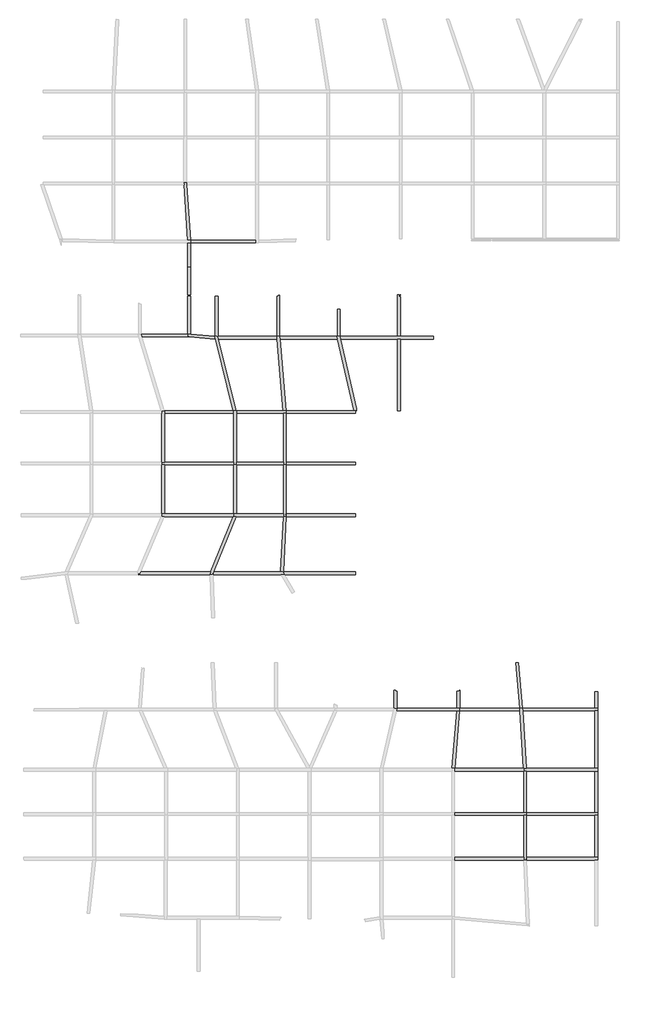
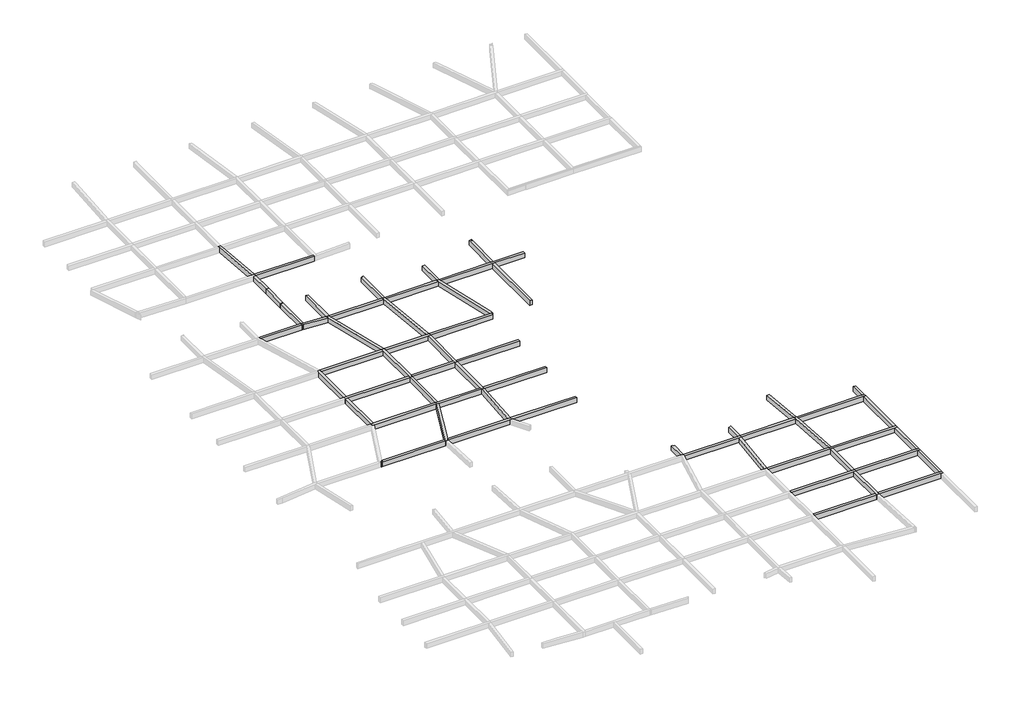
# One storey, part 14 of 15: 57 beams.
"""IFC4 building model written with IfcOpenShell, lengths in millimetres."""

from ifc_helpers import new_model, si_unit, frame, origin, place, context, project, spatial, polyline, outline, extrude, faceted_brep, element, save

model = new_model("IFC4")

# Units and contexts
model_context = context("Model", 3, world=origin())
ifc_project = project(units=[si_unit("LENGTHUNIT", "METRE", prefix="MILLI")], contexts=[model_context])

# Site, building, storey
site = spatial("IfcSite", under=ifc_project)
building = spatial("IfcBuilding", under=site)
storey = spatial("IfcBuildingStorey", under=building, Name="层高", Elevation=3300.0)

# Beams
placement = place(None, origin())
element("IfcBeam", 1, ObjectType="混凝土 - 矩形梁 : KL_beam", at=placement, inside=storey, context=model_context, shape_type="Brep", body=[
    faceted_brep([(295749.8189959, 38242.26105, 3300.0), (295749.8189959, 38542.26105, 3300.0), (295449.8189959, 38542.26105, 3300.0), (287949.8189959, 38542.26105, 3300.0), (287949.8189959, 38242.26105, 3300.0), (295449.8189959, 38242.26105, 3300.0), (295749.8189959, 38242.26105, 2700.0), (287949.8189959, 38242.26105, 2700.0), (295449.8189959, 38242.26105, 2700.0), (295749.8189959, 38542.26105, 2700.0), (287949.8189959, 38542.26105, 2700.0), (295449.8189959, 38542.26105, 2700.0)], [[[0, 1, 2, 3, 4, 5]], [[6, 0, 5, 4, 7, 8]], [[9, 6, 8, 7, 10, 11]], [[1, 9, 11, 10, 3, 2]], [[4, 3, 10, 7]], [[1, 0, 6, 9]]]),
])
element("IfcBeam", 2, ObjectType="混凝土 - 矩形梁 : KL_beam", at=placement, inside=storey, context=model_context, shape_type="Brep", body=[
    faceted_brep([(295449.8189959, 33392.26105, 3300.0), (295456.3366783, 33392.26105, 3300.0), (295749.8189959, 33392.26105, 3300.0), (295749.8189959, 33545.5922638, 3300.0), (295749.8189959, 33692.26105, 3300.0), (295749.8189959, 38242.26105, 3300.0), (295449.8189959, 38242.26105, 3300.0), (295449.8189959, 33692.26105, 3300.0), (295449.8189959, 33392.26105, 2700.0), (295449.8189959, 38242.26105, 2700.0), (295449.8189959, 33692.26105, 2700.0), (295749.8189959, 33392.26105, 2700.0), (295456.3366783, 33392.26105, 2700.0), (295749.8189959, 38242.26105, 2700.0), (295749.8189959, 33692.26105, 2700.0), (295749.8189959, 33545.5922638, 2700.0)], [[[0, 1, 2, 3, 4, 5, 6, 7]], [[8, 0, 7, 6, 9, 10]], [[11, 12, 8, 10, 9, 13, 14, 15]], [[2, 11, 15, 14, 13, 5, 4, 3]], [[6, 5, 13, 9]], [[2, 1, 0, 8, 12, 11]]]),
])
element("IfcBeam", 3, ObjectType="混凝土 - 矩形梁 : KL_beam", at=placement, inside=storey, context=model_context, shape_type="SweptSolid", body=[
    extrude(outline(polyline([(287949.8189959, 33392.26105), (287949.8189959, 33692.26105), (295449.8189959, 33692.26105), (295449.8189959, 33392.26105), (287949.8189959, 33392.26105)])), frame((0.0, 0.0, 2700.0), z_axis=(0.0, 0.0, 1.0), x_axis=(1.0, 0.0, 0.0)), (0.0, 0.0, 1.0), 600.0),
])
element("IfcBeam", 4, ObjectType="混凝土 - 矩形梁 : KL_beam", at=placement, inside=storey, context=model_context, shape_type="Brep", body=[
    faceted_brep([(288493.1023865, 49901.7141002, 3300.0), (288493.1023865, 49901.7141002, 2700.0), (288205.2674175, 49901.7141002, 2700.0), (281663.9582145, 49901.7141002, 2700.0), (281394.6387533, 49901.7141002, 2700.0), (281394.6387533, 49901.7141002, 3300.0), (281663.9582145, 49901.7141002, 3300.0), (288205.2674175, 49901.7141002, 3300.0), (288493.1023865, 49601.7141002, 3300.0), (288192.0287258, 49601.7141002, 3300.0), (281633.2776757, 49601.7141002, 3300.0), (281633.2776757, 49601.7141002, 2700.0), (288192.0287258, 49601.7141002, 2700.0), (288493.1023865, 49601.7141002, 2700.0), (281686.9520176, 49834.2385082, 3300.0), (281686.9520176, 49834.2385082, 2700.0)], [[[0, 1, 2, 3, 4, 5, 6, 7]], [[8, 9, 10, 11, 12, 13]], [[14, 15, 11, 10]], [[15, 14, 5, 4]], [[8, 13, 1, 0]], [[10, 9, 8, 0, 7, 6, 5, 14]], [[13, 12, 11, 15, 4, 3, 2, 1]]]),
])
element("IfcBeam", 5, ObjectType="混凝土 - 矩形梁 : KL_beam", at=placement, inside=storey, context=model_context, shape_type="Brep", body=[
    faceted_brep([(303499.820949, 33392.26105, 3300.0), (303499.820949, 33692.26105, 3300.0), (303199.820949, 33692.26105, 3300.0), (295749.8189959, 33692.26105, 3300.0), (295749.8189959, 33545.5922638, 3300.0), (295756.6327439, 33392.26105, 3300.0), (303199.820949, 33392.26105, 3300.0), (303499.820949, 33392.26105, 2700.0), (295756.6327439, 33392.26105, 2700.0), (303199.820949, 33392.26105, 2700.0), (303499.820949, 33692.26105, 2700.0), (295749.8189959, 33545.5922638, 2700.0), (295749.8189959, 33692.26105, 2700.0), (303199.820949, 33692.26105, 2700.0)], [[[0, 1, 2, 3, 4, 5, 6]], [[7, 0, 6, 5, 8, 9]], [[10, 7, 9, 8, 11, 12, 13]], [[12, 3, 2, 1, 10, 13]], [[3, 12, 11, 4]], [[5, 4, 11, 8]], [[1, 0, 7, 10]]]),
])
element("IfcBeam", 6, ObjectType="混凝土 - 矩形梁 : KL_beam", at=placement, inside=storey, context=model_context, shape_type="Brep", body=[
    faceted_brep([(303499.820949, 38242.26105, 3300.0), (303499.820949, 38542.26105, 3300.0), (303199.820949, 38542.26105, 3300.0), (295749.8189959, 38542.26105, 3300.0), (295749.8189959, 38242.26105, 3300.0), (303199.820949, 38242.26105, 3300.0), (303499.820949, 38242.26105, 2700.0), (295749.8189959, 38242.26105, 2700.0), (303199.820949, 38242.26105, 2700.0), (303499.820949, 38542.26105, 2700.0), (295749.8189959, 38542.26105, 2700.0), (303199.820949, 38542.26105, 2700.0)], [[[0, 1, 2, 3, 4, 5]], [[6, 0, 5, 4, 7, 8]], [[9, 6, 8, 7, 10, 11]], [[1, 9, 11, 10, 3, 2]], [[4, 3, 10, 7]], [[1, 0, 6, 9]]]),
])
element("IfcBeam", 7, ObjectType="混凝土 - 矩形梁 : KL_beam", at=placement, inside=storey, context=model_context, shape_type="Brep", body=[
    faceted_brep([(303499.820949, 43042.26105, 3300.0), (303499.820949, 43342.26105, 3300.0), (303199.820949, 43342.26105, 3300.0), (295740.5303996, 43342.26105, 3300.0), (295449.8189959, 43342.26105, 3300.0), (295449.8189959, 43042.26105, 3300.0), (295749.8189959, 43042.26105, 3300.0), (303199.820949, 43042.26105, 3300.0), (303499.820949, 43042.26105, 2700.0), (295449.8189959, 43042.26105, 2700.0), (295749.8189959, 43042.26105, 2700.0), (303199.820949, 43042.26105, 2700.0), (303499.820949, 43342.26105, 2700.0), (295449.8189959, 43342.26105, 2700.0), (295740.5303996, 43342.26105, 2700.0), (303199.820949, 43342.26105, 2700.0)], [[[0, 1, 2, 3, 4, 5, 6, 7]], [[8, 0, 7, 6, 5, 9, 10, 11]], [[12, 8, 11, 10, 9, 13, 14, 15]], [[1, 12, 15, 14, 13, 4, 3, 2]], [[1, 0, 8, 12]], [[5, 4, 13, 9]]]),
])
element("IfcBeam", 8, ObjectType="混凝土 - 矩形梁 : KL_beam", at=placement, inside=storey, context=model_context, shape_type="SweptSolid", body=[
    extrude(outline(polyline([(303499.820949, 38542.26105), (303199.820949, 38542.26105), (303199.820949, 43042.26105), (303499.820949, 43042.26105), (303499.820949, 38542.26105)])), frame((0.0, 0.0, 2700.0), z_axis=(0.0, 0.0, 1.0), x_axis=(1.0, 0.0, 0.0)), (0.0, 0.0, 1.0), 600.0),
])
element("IfcBeam", 9, ObjectType="混凝土 - 矩形梁 : KL_beam", at=placement, inside=storey, context=model_context, shape_type="SweptSolid", body=[
    extrude(outline(polyline([(295749.8189959, 38542.26105), (295449.8189959, 38542.26105), (295449.8189959, 43042.26105), (295749.8189959, 43042.26105), (295749.8189959, 38542.26105)])), frame((0.0, 0.0, 2700.0), z_axis=(0.0, 0.0, 1.0), x_axis=(1.0, 0.0, 0.0)), (0.0, 0.0, 1.0), 600.0),
])
element("IfcBeam", 10, ObjectType="混凝土 - 矩形梁 : KL_beam", at=placement, inside=storey, context=model_context, shape_type="Brep", body=[
    faceted_brep([(295449.8189959, 43042.26105, 3300.0), (295449.8189959, 43342.26105, 3300.0), (295439.9172438, 43342.26105, 3300.0), (287963.0576876, 43342.26105, 3300.0), (287949.8189959, 43342.26105, 3300.0), (287949.8189959, 43042.26105, 3300.0), (295449.8189959, 43042.26105, 2700.0), (287949.8189959, 43042.26105, 2700.0), (295449.8189959, 43342.26105, 2700.0), (287949.8189959, 43342.26105, 2700.0), (287963.0576876, 43342.26105, 2700.0), (295439.9172438, 43342.26105, 2700.0)], [[[0, 1, 2, 3, 4, 5]], [[6, 0, 5, 7]], [[8, 6, 7, 9, 10, 11]], [[1, 8, 11, 10, 9, 4, 3, 2]], [[1, 0, 6, 8]], [[5, 4, 9, 7]]]),
])
element("IfcBeam", 11, ObjectType="混凝土 - 矩形梁 : KL_beam", at=placement, inside=storey, context=model_context, shape_type="Brep", body=[
    faceted_brep([(288493.1023865, 49601.7141002, 2700.0), (288493.1023865, 49601.7141002, 3300.0), (287963.0576876, 43342.26105, 3300.0), (287963.0576876, 43342.26105, 2700.0), (288192.0287258, 49601.7141002, 3300.0), (288192.0287258, 49601.7141002, 2700.0), (287661.984027, 43342.26105, 3300.0), (287661.984027, 43342.26105, 2700.0), (287949.8189959, 43342.26105, 2700.0), (287949.8189959, 43342.26105, 3300.0)], [[[0, 1, 2, 3]], [[4, 1, 0, 5]], [[6, 7, 8, 3, 2, 9]], [[1, 4, 6, 9, 2]], [[4, 5, 7, 6]], [[5, 0, 3, 8, 7]]]),
])
element("IfcBeam", 12, ObjectType="混凝土 - 矩形梁 : KL_beam", at=placement, inside=storey, context=model_context, shape_type="Brep", body=[
    faceted_brep([(295439.9172438, 43342.26105, 3300.0), (295449.8189959, 43342.26105, 3300.0), (295740.5303996, 43342.26105, 3300.0), (295340.1267819, 49601.7141002, 3300.0), (295320.9364335, 49901.7141002, 3300.0), (295317.6747059, 49901.7141002, 3300.0), (295020.3232776, 49901.7141002, 3300.0), (295039.5136261, 49601.7141002, 3300.0), (295020.3232776, 49901.7141002, 2700.0), (295039.5136261, 49601.7141002, 2700.0), (295439.9172438, 43342.26105, 2700.0), (295740.5303996, 43342.26105, 2700.0), (295449.8189959, 43342.26105, 2700.0), (295317.6747059, 49901.7141002, 2700.0), (295320.9364335, 49901.7141002, 2700.0), (295340.1267819, 49601.7141002, 2700.0)], [[[0, 1, 2, 3, 4, 5, 6, 7]], [[6, 8, 9, 10, 0, 7]], [[11, 12, 10, 9, 8, 13, 14, 15]], [[2, 11, 15, 14, 4, 3]], [[0, 10, 12, 11, 2, 1]], [[6, 5, 4, 14, 13, 8]]]),
])
element("IfcBeam", 13, ObjectType="混凝土 - 矩形梁 : KL_beam", at=placement, inside=storey, context=model_context, shape_type="Brep", body=[
    faceted_brep([(288493.1023865, 49901.7141002, 3300.0), (288493.1023865, 49601.7141002, 3300.0), (295039.5136261, 49601.7141002, 3300.0), (295020.3232776, 49901.7141002, 3300.0), (295016.5287546, 49901.7141002, 3300.0), (288505.2674175, 49901.7141002, 3300.0), (288493.1023865, 49601.7141002, 2700.0), (295039.5136261, 49601.7141002, 2700.0), (288493.1023865, 49901.7141002, 2700.0), (288505.2674175, 49901.7141002, 2700.0), (295016.5287546, 49901.7141002, 2700.0), (295020.3232776, 49901.7141002, 2700.0)], [[[0, 1, 2, 3, 4, 5]], [[1, 6, 7, 2]], [[6, 8, 9, 10, 11, 7]], [[8, 0, 5, 4, 3, 11, 10, 9]], [[1, 0, 8, 6]], [[3, 2, 7, 11]]]),
])
element("IfcBeam", 14, ObjectType="混凝土 - 矩形梁 : KL_beam", at=placement, inside=storey, context=model_context, shape_type="Brep", body=[
    faceted_brep([(295320.9364335, 49901.7141002, 3300.0), (295340.1267819, 49601.7141002, 3300.0), (303199.820949, 49601.7141002, 3300.0), (303499.820949, 49601.7141002, 3300.0), (303499.820949, 49901.7141002, 3300.0), (303199.820949, 49901.7141002, 3300.0), (295340.1267819, 49601.7141002, 2700.0), (303199.820949, 49601.7141002, 2700.0), (303499.820949, 49601.7141002, 2700.0), (295320.9364335, 49901.7141002, 2700.0), (303199.820949, 49901.7141002, 2700.0), (303499.820949, 49901.7141002, 2700.0)], [[[0, 1, 2, 3, 4, 5]], [[1, 6, 7, 8, 3, 2]], [[6, 9, 10, 11, 8, 7]], [[9, 0, 5, 4, 11, 10]], [[1, 0, 9, 6]], [[4, 3, 8, 11]]]),
])
element("IfcBeam", 15, ObjectType="混凝土 - 矩形梁 : KL_beam", at=placement, inside=storey, context=model_context, shape_type="SweptSolid", body=[
    extrude(outline(polyline([(303499.820949, 43342.26105), (303199.820949, 43342.26105), (303199.820949, 49601.7141002), (303499.820949, 49601.7141002), (303499.820949, 43342.26105)])), frame((0.0, 0.0, 2700.0), z_axis=(0.0, 0.0, 1.0), x_axis=(1.0, 0.0, 0.0)), (0.0, 0.0, 1.0), 600.0),
])
element("IfcBeam", 16, ObjectType="混凝土 - 矩形梁 : KL_beam", at=placement, inside=storey, context=model_context, shape_type="SweptSolid", body=[
    extrude(outline(polyline([(303499.820949, 49901.7141002), (303199.820949, 49901.7141002), (303199.820949, 51682.3314613), (303499.820949, 51682.3314613), (303499.820949, 49901.7141002)])), frame((0.0, 0.0, 2700.0), z_axis=(0.0, 0.0, 1.0), x_axis=(1.0, 0.0, 0.0)), (0.0, 0.0, 1.0), 600.0),
])
element("IfcBeam", 17, ObjectType="混凝土 - 矩形梁 : KL_beam", at=placement, inside=storey, context=model_context, shape_type="Brep", body=[
    faceted_brep([(281363.9582145, 51842.0227808, 2700.0), (281363.9582145, 51842.0227808, 3300.0), (281540.2344711, 51842.0227808, 3300.0), (281540.2344711, 51842.0227808, 2700.0), (281363.9582145, 49901.7141002, 3300.0), (281394.6387533, 49901.7141002, 3300.0), (281663.9582145, 49901.7141002, 3300.0), (281663.9582145, 51732.3246977, 3300.0), (281540.2344711, 51732.3246977, 3300.0), (281663.9582145, 49901.7141002, 2700.0), (281663.9582145, 51732.3246977, 2700.0), (281363.9582145, 49901.7141002, 2700.0), (281540.2344711, 51732.3246977, 2700.0), (281394.6387533, 49901.7141002, 2700.0)], [[[0, 1, 2, 3]], [[1, 4, 5, 6, 7, 8, 2]], [[6, 9, 10, 7]], [[11, 0, 3, 12, 10, 9, 13]], [[1, 0, 11, 4]], [[4, 11, 13, 9, 6, 5]], [[12, 8, 7, 10]], [[8, 12, 3, 2]]]),
])
element("IfcBeam", 18, ObjectType="混凝土 - 矩形梁 : KL_beam", at=placement, inside=storey, context=model_context, shape_type="Brep", body=[
    faceted_brep([(288205.2674175, 49901.7141002, 3300.0), (288493.1023865, 49901.7141002, 3300.0), (288505.2674175, 49901.7141002, 3300.0), (288505.2674175, 51852.3246977, 3300.0), (288460.2344711, 51852.3246977, 3300.0), (288460.2344711, 51732.3246977, 3300.0), (288340.2344711, 51732.3246977, 3300.0), (288205.2674175, 51732.3246977, 3300.0), (288505.2674175, 49901.7141002, 2700.0), (288505.2674175, 51852.3246977, 2700.0), (288493.1023865, 49901.7141002, 2700.0), (288205.2674175, 49901.7141002, 2700.0), (288205.2674175, 51732.3246977, 2700.0), (288460.2344711, 51732.3246977, 2700.0), (288460.2344711, 51852.3246977, 2700.0)], [[[0, 1, 2, 3, 4, 5, 6, 7]], [[2, 8, 9, 3]], [[8, 10, 11, 12, 13, 14, 9]], [[11, 0, 7, 12]], [[0, 11, 10, 8, 2, 1]], [[3, 9, 14, 4]], [[5, 13, 12, 7, 6]], [[13, 5, 4, 14]]]),
])
element("IfcBeam", 19, ObjectType="混凝土 - 矩形梁 : KL_beam", at=placement, inside=storey, context=model_context, shape_type="Brep", body=[
    faceted_brep([(295016.5287546, 49901.7141002, 3300.0), (295020.3232776, 49901.7141002, 3300.0), (295317.6747059, 49901.7141002, 3300.0), (294886.3021743, 54832.3246977, 3300.0), (294585.1562231, 54832.3246977, 3300.0), (295317.6747059, 49901.7141002, 2700.0), (294886.3021743, 54832.3246977, 2700.0), (295020.3232776, 49901.7141002, 2700.0), (295016.5287546, 49901.7141002, 2700.0), (294585.1562231, 54832.3246977, 2700.0)], [[[0, 1, 2, 3, 4]], [[2, 5, 6, 3]], [[5, 7, 8, 9, 6]], [[8, 0, 4, 9]], [[5, 2, 1, 0, 8, 7]], [[4, 3, 6, 9]]]),
])
element("IfcBeam", 20, ObjectType="混凝土 - 矩形梁 : KL_beam", at=placement, inside=storey, context=model_context, shape_type="SweptSolid", body=[
    extrude(outline(polyline([(303499.820949, 33692.26105), (303199.820949, 33692.26105), (303199.820949, 38242.26105), (303499.820949, 38242.26105), (303499.820949, 33692.26105)])), frame((0.0, 0.0, 2700.0), z_axis=(0.0, 0.0, 1.0), x_axis=(1.0, 0.0, 0.0)), (0.0, 0.0, 1.0), 600.0),
])
element("IfcBeam", 21, ObjectType="混凝土 - 矩形梁 : KL_beam", at=placement, inside=storey, context=model_context, shape_type="SweptSolid", body=[
    extrude(outline(polyline([(259271.6890495, 97741.6486698), (258971.6890495, 97741.6486698), (258971.6890495, 100391.6486698), (259271.6890495, 100391.6486698), (259271.6890495, 97741.6486698)])), frame((0.0, 0.0, 2700.0), z_axis=(0.0, 0.0, 1.0), x_axis=(1.0, 0.0, 0.0)), (0.0, 0.0, 1.0), 600.0),
])
element("IfcBeam", 22, ObjectType="混凝土 - 矩形梁 : KL_beam", at=placement, inside=storey, context=model_context, shape_type="Brep", body=[
    faceted_brep([(263949.8021775, 76292.0126466, 3300.0), (264249.8021775, 76292.0126466, 3300.0), (264249.8021775, 76592.0126466, 3300.0), (264249.8021775, 81892.0126467, 3300.0), (264249.8021775, 82192.0126467, 3300.0), (264216.9950214, 82192.0126467, 3300.0), (263949.8021775, 82192.0126467, 3300.0), (263949.8021775, 81892.0126467, 3300.0), (263949.8021775, 76592.0126466, 3300.0), (263949.8021775, 76292.0126466, 2700.0), (263949.8021775, 82192.0126467, 2700.0), (263949.8021775, 81892.0126467, 2700.0), (263949.8021775, 76592.0126466, 2700.0), (264249.8021775, 76292.0126466, 2700.0), (264216.9950214, 82192.0126467, 2700.0), (264249.8021775, 82192.0126467, 2700.0), (264249.8021775, 81892.0126467, 2700.0), (264249.8021775, 76592.0126466, 2700.0)], [[[0, 1, 2, 3, 4, 5, 6, 7, 8]], [[9, 0, 8, 7, 6, 10, 11, 12]], [[13, 9, 12, 11, 10, 14, 15, 16, 17]], [[1, 13, 17, 16, 15, 4, 3, 2]], [[1, 0, 9, 13]], [[6, 5, 4, 15, 14, 10]]]),
])
element("IfcBeam", 23, ObjectType="混凝土 - 矩形梁 : KL_beam", at=placement, inside=storey, context=model_context, shape_type="Brep", body=[
    faceted_brep([(256149.8021771, 76592.0126466, 3300.0), (256149.8021771, 76302.5702379, 3300.0), (256149.8021771, 76292.0126466, 3300.0), (256449.8021771, 76292.0126466, 3300.0), (263949.8021775, 76292.0126466, 3300.0), (263949.8021775, 76592.0126466, 3300.0), (256449.8021771, 76592.0126466, 3300.0), (256149.8021771, 76592.0126466, 2700.0), (263949.8021775, 76592.0126466, 2700.0), (256449.8021771, 76592.0126466, 2700.0), (256149.8021771, 76292.0126466, 2700.0), (256149.8021771, 76302.5702379, 2700.0), (263949.8021775, 76292.0126466, 2700.0), (256449.8021771, 76292.0126466, 2700.0)], [[[0, 1, 2, 3, 4, 5, 6]], [[7, 0, 6, 5, 8, 9]], [[10, 11, 7, 9, 8, 12, 13]], [[2, 10, 13, 12, 4, 3]], [[5, 4, 12, 8]], [[2, 1, 0, 7, 11, 10]]]),
])
element("IfcBeam", 24, ObjectType="混凝土 - 矩形梁 : KL_beam", at=placement, inside=storey, context=model_context, shape_type="Brep", body=[
    faceted_brep([(256449.8021771, 82192.0126467, 3300.0), (256410.7963384, 82192.0126467, 3300.0), (256149.8021771, 82192.0126467, 3300.0), (256149.8021771, 82019.5949965, 3300.0), (256149.8021771, 81897.4603606, 3300.0), (256149.8021771, 76602.5702379, 3300.0), (256149.8021771, 76592.0126466, 3300.0), (256449.8021771, 76592.0126466, 3300.0), (256449.8021771, 81892.0126467, 3300.0), (256149.8021771, 82192.0126467, 2700.0), (256149.8021771, 82019.5949965, 2700.0), (256149.8021771, 81897.4603606, 2700.0), (256149.8021771, 76602.5702379, 2700.0), (256149.8021771, 76592.0126466, 2700.0), (256410.7963384, 82192.0126467, 2700.0), (256449.8021771, 82192.0126467, 2700.0), (256449.8021771, 81892.0126467, 2700.0), (256449.8021771, 76592.0126466, 2700.0)], [[[0, 1, 2, 3, 4, 5, 6, 7, 8]], [[2, 9, 10, 11, 12, 13, 6, 5, 4, 3]], [[9, 14, 15, 16, 17, 13, 12, 11, 10]], [[15, 0, 8, 7, 17, 16]], [[7, 6, 13, 17]], [[2, 1, 0, 15, 14, 9]]]),
])
element("IfcBeam", 25, ObjectType="混凝土 - 矩形梁 : KL_beam", at=placement, inside=storey, context=model_context, shape_type="Brep", body=[
    faceted_brep([(263949.8021775, 81892.0126467, 3300.0), (263949.8021775, 82192.0126467, 3300.0), (263907.8109326, 82192.0126467, 3300.0), (256449.8021771, 82192.0126467, 3300.0), (256449.8021771, 81892.0126467, 3300.0), (263949.8021775, 81892.0126467, 2700.0), (256449.8021771, 81892.0126467, 2700.0), (263949.8021775, 82192.0126467, 2700.0), (256449.8021771, 82192.0126467, 2700.0), (263907.8109326, 82192.0126467, 2700.0)], [[[0, 1, 2, 3, 4]], [[5, 0, 4, 6]], [[7, 5, 6, 8, 9]], [[1, 7, 9, 8, 3, 2]], [[1, 0, 5, 7]], [[4, 3, 8, 6]]]),
])
element("IfcBeam", 26, ObjectType="混凝土 - 矩形梁 : KL_beam", at=placement, inside=storey, context=model_context, shape_type="Brep", body=[
    faceted_brep([(264249.8021775, 82192.0126467, 3300.0), (264249.8021775, 81892.0126467, 3300.0), (269354.7419848, 81892.0126467, 3300.0), (269654.7419848, 81892.0126467, 3300.0), (269654.7419848, 82192.0126467, 3300.0), (269642.1916609, 82192.0126467, 3300.0), (269341.0457096, 82192.0126467, 3300.0), (264249.8021775, 81892.0126467, 2700.0), (269354.7419848, 81892.0126467, 2700.0), (269654.7419848, 81892.0126467, 2700.0), (264249.8021775, 82192.0126467, 2700.0), (269341.0457096, 82192.0126467, 2700.0), (269642.1916609, 82192.0126467, 2700.0), (269654.7419848, 82192.0126467, 2700.0)], [[[0, 1, 2, 3, 4, 5, 6]], [[1, 7, 8, 9, 3, 2]], [[7, 10, 11, 12, 13, 9, 8]], [[10, 0, 6, 5, 4, 13, 12, 11]], [[1, 0, 10, 7]], [[4, 3, 9, 13]]]),
])
element("IfcBeam", 27, ObjectType="混凝土 - 矩形梁 : KL_beam", at=placement, inside=storey, context=model_context, shape_type="Brep", body=[
    faceted_brep([(269354.7419848, 76292.0126466, 3300.0), (269654.7419848, 76292.0126466, 3300.0), (269654.7419848, 76592.0126466, 3300.0), (269654.7419848, 81892.0126467, 3300.0), (269354.7419848, 81892.0126467, 3300.0), (269354.7419848, 76592.0126466, 3300.0), (269354.7419848, 76292.0126466, 2700.0), (269354.7419848, 81892.0126467, 2700.0), (269354.7419848, 76592.0126466, 2700.0), (269654.7419848, 76292.0126466, 2700.0), (269654.7419848, 81892.0126467, 2700.0), (269654.7419848, 76592.0126466, 2700.0)], [[[0, 1, 2, 3, 4, 5]], [[6, 0, 5, 4, 7, 8]], [[9, 6, 8, 7, 10, 11]], [[1, 9, 11, 10, 3, 2]], [[4, 3, 10, 7]], [[1, 0, 6, 9]]]),
])
element("IfcBeam", 28, ObjectType="混凝土 - 矩形梁 : KL_beam", at=placement, inside=storey, context=model_context, shape_type="SweptSolid", body=[
    extrude(outline(polyline([(264249.8021775, 76292.0126466), (264249.8021775, 76592.0126466), (269354.7419848, 76592.0126466), (269354.7419848, 76292.0126466), (264249.8021775, 76292.0126466)])), frame((0.0, 0.0, 2700.0), z_axis=(0.0, 0.0, 1.0), x_axis=(1.0, 0.0, 0.0)), (0.0, 0.0, 1.0), 600.0),
])
element("IfcBeam", 29, ObjectType="混凝土 - 矩形梁 : KL_beam", at=placement, inside=storey, context=model_context, shape_type="Brep", body=[
    faceted_brep([(269354.7419848, 70692.0126466, 3300.0), (269647.6593001, 70692.0126466, 3300.0), (269654.7419848, 70692.0126466, 3300.0), (269654.7419848, 70838.3856753, 3300.0), (269654.7419848, 70992.0126466, 3300.0), (269654.7419848, 76292.0126466, 3300.0), (269354.7419848, 76292.0126466, 3300.0), (269354.7419848, 70992.0126466, 3300.0), (269354.7419848, 70692.0126466, 2700.0), (269354.7419848, 76292.0126466, 2700.0), (269354.7419848, 70992.0126466, 2700.0), (269654.7419848, 70692.0126466, 2700.0), (269647.6593001, 70692.0126466, 2700.0), (269654.7419848, 76292.0126466, 2700.0), (269654.7419848, 70992.0126466, 2700.0), (269654.7419848, 70838.3856753, 2700.0)], [[[0, 1, 2, 3, 4, 5, 6, 7]], [[8, 0, 7, 6, 9, 10]], [[11, 12, 8, 10, 9, 13, 14, 15]], [[2, 11, 15, 14, 13, 5, 4, 3]], [[6, 5, 13, 9]], [[2, 1, 0, 8, 12, 11]]]),
])
element("IfcBeam", 30, ObjectType="混凝土 - 矩形梁 : KL_beam", at=placement, inside=storey, context=model_context, shape_type="Brep", body=[
    faceted_brep([(263949.8021775, 70992.0126466, 3300.0), (263949.8021775, 70692.0126466, 3300.0), (264200.978455, 70692.0126466, 3300.0), (269347.308297, 70692.0126466, 3300.0), (269354.7419848, 70692.0126466, 3300.0), (269354.7419848, 70992.0126466, 3300.0), (264249.8021775, 70992.0126466, 3300.0), (263949.8021775, 70992.0126466, 2700.0), (269354.7419848, 70992.0126466, 2700.0), (264249.8021775, 70992.0126466, 2700.0), (263949.8021775, 70692.0126466, 2700.0), (269354.7419848, 70692.0126466, 2700.0), (269347.308297, 70692.0126466, 2700.0), (264200.978455, 70692.0126466, 2700.0)], [[[0, 1, 2, 3, 4, 5, 6]], [[7, 0, 6, 5, 8, 9]], [[10, 7, 9, 8, 11, 12, 13]], [[1, 10, 13, 12, 11, 4, 3, 2]], [[5, 4, 11, 8]], [[1, 0, 7, 10]]]),
])
element("IfcBeam", 31, ObjectType="混凝土 - 矩形梁 : KL_beam", at=placement, inside=storey, context=model_context, shape_type="SweptSolid", body=[
    extrude(outline(polyline([(263949.8021775, 76292.0126466), (264249.8021775, 76292.0126466), (264249.8021775, 70992.0126466), (263949.8021775, 70992.0126466), (263949.8021775, 76292.0126466)])), frame((0.0, 0.0, 2700.0), z_axis=(0.0, 0.0, 1.0), x_axis=(1.0, 0.0, 0.0)), (0.0, 0.0, 1.0), 600.0),
])
element("IfcBeam", 32, ObjectType="混凝土 - 矩形梁 : KL_beam", at=placement, inside=storey, context=model_context, shape_type="Brep", body=[
    faceted_brep([(256149.8021771, 70992.0126466, 3300.0), (256149.8021771, 70872.8035797, 3300.0), (256149.8021771, 70692.0126466, 3300.0), (256398.7084648, 70692.0126466, 3300.0), (263877.4180322, 70692.0126466, 3300.0), (263949.8021775, 70692.0126466, 3300.0), (263949.8021775, 70992.0126466, 3300.0), (256449.8021771, 70992.0126466, 3300.0), (256149.8021771, 70692.0126466, 2700.0), (256398.7084648, 70692.0126466, 2700.0), (263877.4180322, 70692.0126466, 2700.0), (263949.8021775, 70692.0126466, 2700.0), (256149.8021771, 70872.8035797, 2700.0), (256149.8021771, 70992.0126466, 2700.0), (256449.8021771, 70992.0126466, 2700.0), (263949.8021775, 70992.0126466, 2700.0)], [[[0, 1, 2, 3, 4, 5, 6, 7]], [[2, 8, 9, 10, 11, 5, 4, 3]], [[8, 12, 13, 14, 15, 11, 10, 9]], [[13, 0, 7, 6, 15, 14]], [[6, 5, 11, 15]], [[2, 1, 0, 13, 12, 8]]]),
])
element("IfcBeam", 33, ObjectType="混凝土 - 矩形梁 : KL_beam", at=placement, inside=storey, context=model_context, shape_type="SweptSolid", body=[
    extrude(outline(polyline([(256149.8021771, 76292.0126466), (256449.8021771, 76292.0126466), (256449.8021771, 70992.0126466), (256149.8021771, 70992.0126466), (256149.8021771, 76292.0126466)])), frame((0.0, 0.0, 2700.0), z_axis=(0.0, 0.0, 1.0), x_axis=(1.0, 0.0, 0.0)), (0.0, 0.0, 1.0), 600.0),
])
element("IfcBeam", 34, ObjectType="混凝土 - 矩形梁 : KL_beam", at=placement, inside=storey, context=model_context, shape_type="Brep", body=[
    faceted_brep([(264200.978455, 70692.0126466, 3300.0), (263949.8021775, 70692.0126466, 3300.0), (263877.4180322, 70692.0126466, 3300.0), (261453.2606772, 64692.0126466, 3300.0), (261332.0528094, 64392.0126466, 3300.0), (261409.5836385, 64392.0126466, 3300.0), (261655.6132322, 64392.0126466, 3300.0), (261705.4582963, 64515.3835094, 3300.0), (261776.8211, 64692.0126466, 3300.0), (261332.0528094, 64392.0126466, 2700.0), (263877.4180322, 70692.0126466, 2700.0), (261453.2606772, 64692.0126466, 2700.0), (263949.8021775, 70692.0126466, 2700.0), (264200.978455, 70692.0126466, 2700.0), (261776.8211, 64692.0126466, 2700.0), (261705.4582963, 64515.3835094, 2700.0), (261655.6132322, 64392.0126466, 2700.0), (261409.5836385, 64392.0126466, 2700.0)], [[[0, 1, 2, 3, 4, 5, 6, 7, 8]], [[9, 4, 3, 2, 10, 11]], [[10, 12, 13, 14, 15, 16, 17, 9, 11]], [[13, 0, 8, 7, 6, 16, 15, 14]], [[0, 13, 12, 10, 2, 1]], [[6, 5, 4, 9, 17, 16]]]),
])
element("IfcBeam", 35, ObjectType="混凝土 - 矩形梁 : KL_beam", at=placement, inside=storey, context=model_context, shape_type="SweptSolid", body=[
    extrude(outline(polyline([(261453.2606772, 64692.0126466), (261332.0528094, 64392.0126466), (253809.5875713, 64392.0126466), (253809.5875713, 64542.2610502), (253762.8884968, 64542.2610502), (253827.0729182, 64692.0126466), (261453.2606772, 64692.0126466)])), frame((0.0, 0.0, 2700.0), z_axis=(0.0, 0.0, 1.0), x_axis=(1.0, 0.0, 0.0)), (0.0, 0.0, 1.0), 600.0),
    extrude(outline(polyline([(253599.5848532, 64392.0126466), (253599.5848532, 64542.165729), (253689.5875713, 64503.5900308), (253689.5875713, 64392.0126466), (253599.5848532, 64392.0126466)])), frame((0.0, 0.0, 2700.0), z_axis=(0.0, 0.0, 1.0), x_axis=(1.0, 0.0, 0.0)), (0.0, 0.0, 1.0), 600.0),
])
element("IfcBeam", 36, ObjectType="混凝土 - 矩形梁 : KL_beam", at=placement, inside=storey, context=model_context, shape_type="Brep", body=[
    faceted_brep([(269459.7057839, 64392.0126466, 3300.0), (269351.8545261, 64578.8165049, 3300.0), (269286.5007032, 64692.0126466, 3300.0), (269056.9808475, 64692.0126466, 3300.0), (261776.8211, 64692.0126466, 3300.0), (261705.4582963, 64515.3835094, 3300.0), (261709.7665018, 64392.0126466, 3300.0), (269113.2956224, 64392.0126466, 3300.0), (269459.7057839, 64392.0126466, 2700.0), (261709.7665018, 64392.0126466, 2700.0), (269113.2956224, 64392.0126466, 2700.0), (269286.5007032, 64692.0126466, 2700.0), (269351.8545261, 64578.8165049, 2700.0), (261705.4582963, 64515.3835094, 2700.0), (261776.8211, 64692.0126466, 2700.0), (269056.9808475, 64692.0126466, 2700.0)], [[[0, 1, 2, 3, 4, 5, 6, 7]], [[8, 0, 7, 6, 9, 10]], [[11, 12, 8, 10, 9, 13, 14, 15]], [[14, 4, 3, 2, 11, 15]], [[4, 14, 13, 5]], [[6, 5, 13, 9]], [[2, 1, 0, 8, 12, 11]]]),
])
element("IfcBeam", 37, ObjectType="混凝土 - 矩形梁 : KL_beam", at=placement, inside=storey, context=model_context, shape_type="Brep", body=[
    faceted_brep([(269647.6593001, 70692.0126466, 3300.0), (269354.7419848, 70692.0126466, 3300.0), (269347.308297, 70692.0126466, 3300.0), (269056.9808475, 64692.0126466, 3300.0), (269286.5007032, 64692.0126466, 3300.0), (269351.8545261, 64578.8165049, 3300.0), (269357.3318506, 64692.0126466, 3300.0), (269347.308297, 70692.0126466, 2700.0), (269056.9808475, 64692.0126466, 2700.0), (269354.7419848, 70692.0126466, 2700.0), (269647.6593001, 70692.0126466, 2700.0), (269357.3318506, 64692.0126466, 2700.0), (269351.8545261, 64578.8165049, 2700.0), (269286.5007032, 64692.0126466, 2700.0)], [[[0, 1, 2, 3, 4, 5, 6]], [[2, 7, 8, 3]], [[7, 9, 10, 11, 12, 13, 8]], [[10, 0, 6, 5, 12, 11]], [[0, 10, 9, 7, 2, 1]], [[13, 4, 3, 8]], [[4, 13, 12, 5]]]),
    faceted_brep([(269654.7419848, 70992.0126466, 2700.0), (269654.7419848, 70992.0126466, 3300.0), (269662.1756726, 70992.0126466, 3300.0), (269662.1756726, 70992.0126466, 2700.0), (269654.7419848, 70838.3856753, 3300.0), (269654.7419848, 70838.3856753, 2700.0)], [[[0, 1, 2, 3]], [[4, 1, 0, 5]], [[4, 2, 1]], [[3, 5, 0]], [[2, 4, 5, 3]]]),
])
element("IfcBeam", 38, ObjectType="混凝土 - 矩形梁 : KL_beam", at=placement, inside=storey, context=model_context, shape_type="SweptSolid", body=[
    extrude(outline(polyline([(269654.7419848, 70692.0126466), (269654.7419848, 70838.3856753), (269662.1756726, 70992.0126466), (277178.9838503, 70992.0126466), (277178.9838503, 70692.0126466), (269654.7419848, 70692.0126466)])), frame((0.0, 0.0, 2700.0), z_axis=(0.0, 0.0, 1.0), x_axis=(1.0, 0.0, 0.0)), (0.0, 0.0, 1.0), 600.0),
])
element("IfcBeam", 39, ObjectType="混凝土 - 矩形梁 : KL_beam", at=placement, inside=storey, context=model_context, shape_type="SweptSolid", body=[
    extrude(outline(polyline([(269459.7057839, 64392.0126466), (269351.8545261, 64578.8165049), (269357.3318506, 64692.0126466), (277178.9838503, 64692.0126466), (277178.9838503, 64392.0126466), (269459.7057839, 64392.0126466)])), frame((0.0, 0.0, 2700.0), z_axis=(0.0, 0.0, 1.0), x_axis=(1.0, 0.0, 0.0)), (0.0, 0.0, 1.0), 600.0),
])
element("IfcBeam", 40, ObjectType="混凝土 - 矩形梁 : KL_beam", at=placement, inside=storey, context=model_context, shape_type="SweptSolid", body=[
    extrude(outline(polyline([(269654.7419848, 76292.0126466), (269654.7419848, 76592.0126466), (277178.9838503, 76592.0126466), (277178.9838503, 76292.0126466), (269654.7419848, 76292.0126466)])), frame((0.0, 0.0, 2700.0), z_axis=(0.0, 0.0, 1.0), x_axis=(1.0, 0.0, 0.0)), (0.0, 0.0, 1.0), 600.0),
])
element("IfcBeam", 41, ObjectType="混凝土 - 矩形梁 : KL_beam", at=placement, inside=storey, context=model_context, shape_type="Brep", body=[
    faceted_brep([(269654.7419848, 82192.0126467, 3300.0), (269654.7419848, 81892.0126467, 3300.0), (277178.9838503, 81892.0126467, 3300.0), (277178.9838503, 82154.5735496, 3300.0), (277298.9838503, 82154.5735496, 3300.0), (277298.9838503, 82192.0126467, 3300.0), (277039.5877268, 82192.0126467, 3300.0), (269654.7419848, 81892.0126467, 2700.0), (277178.9838503, 81892.0126467, 2700.0), (269654.7419848, 82192.0126467, 2700.0), (277039.5877268, 82192.0126467, 2700.0), (277298.9838503, 82192.0126467, 2700.0), (277298.9838503, 82154.5735496, 2700.0), (277178.9838503, 82154.5735496, 2700.0)], [[[0, 1, 2, 3, 4, 5, 6]], [[1, 7, 8, 2]], [[7, 9, 10, 11, 12, 13, 8]], [[9, 0, 6, 5, 11, 10]], [[1, 0, 9, 7]], [[11, 5, 4, 12]], [[13, 3, 2, 8]], [[3, 13, 12, 4]]]),
])
element("IfcBeam", 42, ObjectType="混凝土 - 矩形梁 : KL_beam", at=placement, inside=storey, context=model_context, shape_type="Brep", body=[
    faceted_brep([(269341.0457096, 82192.0126467, 3300.0), (269354.7419848, 82192.0126467, 3300.0), (269642.1916609, 82192.0126467, 3300.0), (268963.9401389, 89944.4630172, 3300.0), (268937.6935399, 90244.4630172, 3300.0), (268650.2438638, 90244.4630172, 3300.0), (268636.5475886, 90244.4630172, 3300.0), (268662.7941877, 89944.4630172, 3300.0), (269642.1916609, 82192.0126467, 2700.0), (268963.9401389, 89944.4630172, 2700.0), (268937.6935399, 90244.4630172, 2700.0), (269354.7419848, 82192.0126467, 2700.0), (269341.0457096, 82192.0126467, 2700.0), (268662.7941877, 89944.4630172, 2700.0), (268636.5475886, 90244.4630172, 2700.0), (268650.2438638, 90244.4630172, 2700.0)], [[[0, 1, 2, 3, 4, 5, 6, 7]], [[2, 8, 9, 10, 4, 3]], [[8, 11, 12, 13, 14, 15, 10, 9]], [[12, 0, 7, 6, 14, 13]], [[8, 2, 1, 0, 12, 11]], [[6, 5, 4, 10, 15, 14]]]),
])
element("IfcBeam", 43, ObjectType="混凝土 - 矩形梁 : KL_beam", at=placement, inside=storey, context=model_context, shape_type="Brep", body=[
    faceted_brep([(275488.424308, 90244.4630172, 3300.0), (275219.1089205, 90244.4630172, 3300.0), (275180.5330757, 90244.4630172, 3300.0), (275249.793533, 89944.4630172, 3300.0), (277039.5877268, 82192.0126467, 3300.0), (277298.9838503, 82192.0126467, 3300.0), (277298.9838503, 82402.0680408, 3300.0), (275557.6847654, 89944.4630172, 3300.0), (275488.424308, 90244.4630172, 2700.0), (277298.9838503, 82402.0680408, 2700.0), (275557.6847654, 89944.4630172, 2700.0), (275180.5330757, 90244.4630172, 2700.0), (275219.1089205, 90244.4630172, 2700.0), (277298.9838503, 82192.0126467, 2700.0), (277039.5877268, 82192.0126467, 2700.0), (275249.793533, 89944.4630172, 2700.0)], [[[0, 1, 2, 3, 4, 5, 6, 7]], [[8, 0, 7, 6, 9, 10]], [[11, 12, 8, 10, 9, 13, 14, 15]], [[2, 11, 15, 14, 4, 3]], [[5, 4, 14, 13]], [[2, 1, 0, 8, 12, 11]], [[9, 6, 5, 13]]]),
])
element("IfcBeam", 44, ObjectType="混凝土 - 矩形梁 : KL_beam", at=placement, inside=storey, context=model_context, shape_type="Brep", body=[
    faceted_brep([(263907.8109326, 82192.0126467, 3300.0), (263949.8021775, 82192.0126467, 3300.0), (264216.9950214, 82192.0126467, 3300.0), (262284.0920534, 89944.4630172, 3300.0), (262211.647044, 90235.0240798, 3300.0), (262098.3376847, 90244.4630172, 3300.0), (261942.1008086, 90257.4779182, 3300.0), (261895.9051179, 90261.3261284, 3300.0), (261972.5545732, 89953.9019546, 3300.0), (264216.9950214, 82192.0126467, 2700.0), (262284.0920534, 89944.4630172, 2700.0), (262211.647044, 90235.0240798, 2700.0), (263949.8021775, 82192.0126467, 2700.0), (263907.8109326, 82192.0126467, 2700.0), (261972.5545732, 89953.9019546, 2700.0), (261895.9051179, 90261.3261284, 2700.0), (261942.1008086, 90257.4779182, 2700.0), (262098.3376847, 90244.4630172, 2700.0)], [[[0, 1, 2, 3, 4, 5, 6, 7, 8]], [[2, 9, 10, 11, 4, 3]], [[9, 12, 13, 14, 15, 16, 17, 11, 10]], [[13, 0, 8, 7, 15, 14]], [[9, 2, 1, 0, 13, 12]], [[7, 6, 5, 4, 11, 17, 16, 15]]]),
])
element("IfcBeam", 45, ObjectType="混凝土 - 矩形梁 : KL_beam", at=placement, inside=storey, context=model_context, shape_type="Brep", body=[
    faceted_brep([(258971.6890495, 90504.9202371, 3300.0), (258971.6890495, 90491.9053361, 3300.0), (258971.6890495, 90203.8811441, 3300.0), (259115.4521735, 90191.9053361, 3300.0), (261972.5545732, 89953.9019546, 3300.0), (261895.9051179, 90261.3261284, 3300.0), (259271.6890495, 90479.9295282, 3300.0), (258971.6890495, 90203.8811441, 2700.0), (259115.4521735, 90191.9053361, 2700.0), (261972.5545732, 89953.9019546, 2700.0), (258971.6890495, 90491.9053361, 2700.0), (258971.6890495, 90504.9202371, 2700.0), (259271.6890495, 90479.9295282, 2700.0), (261895.9051179, 90261.3261284, 2700.0)], [[[0, 1, 2, 3, 4, 5, 6]], [[2, 7, 8, 9, 4, 3]], [[7, 10, 11, 12, 13, 9, 8]], [[11, 0, 6, 5, 13, 12]], [[5, 4, 9, 13]], [[2, 1, 0, 11, 10, 7]]]),
])
element("IfcBeam", 46, ObjectType="混凝土 - 矩形梁 : KL_beam", at=placement, inside=storey, context=model_context, shape_type="Brep", body=[
    faceted_brep([(268662.7941877, 89944.4630172, 3300.0), (268636.5475886, 90244.4630172, 3300.0), (262242.1008086, 90244.4630172, 3300.0), (262098.3376847, 90244.4630172, 3300.0), (262211.647044, 90235.0240798, 3300.0), (262284.0920534, 89944.4630172, 3300.0), (268662.7941877, 89944.4630172, 2700.0), (262284.0920534, 89944.4630172, 2700.0), (268636.5475886, 90244.4630172, 2700.0), (262211.647044, 90235.0240798, 2700.0), (262098.3376847, 90244.4630172, 2700.0), (262242.1008086, 90244.4630172, 2700.0)], [[[0, 1, 2, 3, 4, 5]], [[6, 0, 5, 7]], [[8, 6, 7, 9, 10, 11]], [[1, 8, 11, 10, 3, 2]], [[1, 0, 6, 8]], [[4, 9, 7, 5]], [[9, 4, 3, 10]]]),
])
element("IfcBeam", 47, ObjectType="混凝土 - 矩形梁 : KL_beam", at=placement, inside=storey, context=model_context, shape_type="Brep", body=[
    faceted_brep([(268937.6935399, 90244.4630172, 3300.0), (268963.9401389, 89944.4630172, 3300.0), (275249.793533, 89944.4630172, 3300.0), (275180.5330757, 90244.4630172, 3300.0), (268950.2438638, 90244.4630172, 3300.0), (268963.9401389, 89944.4630172, 2700.0), (275249.793533, 89944.4630172, 2700.0), (268937.6935399, 90244.4630172, 2700.0), (268950.2438638, 90244.4630172, 2700.0), (275180.5330757, 90244.4630172, 2700.0)], [[[0, 1, 2, 3, 4]], [[1, 5, 6, 2]], [[5, 7, 8, 9, 6]], [[7, 0, 4, 3, 9, 8]], [[1, 0, 7, 5]], [[3, 2, 6, 9]]]),
])
element("IfcBeam", 48, ObjectType="混凝土 - 矩形梁 : KL_beam", at=placement, inside=storey, context=model_context, shape_type="SweptSolid", body=[
    extrude(outline(polyline([(258971.6890495, 97741.6486698), (259271.6890495, 97741.6486698), (259271.6890495, 94749.6848758), (258971.6890495, 94749.6848758), (258971.6890495, 97741.6486698)])), frame((0.0, 0.0, 2700.0), z_axis=(0.0, 0.0, 1.0), x_axis=(1.0, 0.0, 0.0)), (0.0, 0.0, 1.0), 600.0),
    extrude(outline(polyline([(259271.6890495, 90479.9295282), (258971.6890495, 90504.9202371), (258971.6890495, 94629.6848758), (259271.6890495, 94629.6848758), (259271.6890495, 90479.9295282)])), frame((0.0, 0.0, 2700.0), z_axis=(0.0, 0.0, 1.0), x_axis=(1.0, 0.0, 0.0)), (0.0, 0.0, 1.0), 600.0),
])
element("IfcBeam", 49, ObjectType="混凝土 - 矩形梁 : KL_beam", at=placement, inside=storey, context=model_context, shape_type="Brep", body=[
    faceted_brep([(258521.7581821, 106970.7217277, 3300.0), (258541.2728714, 106691.6486698, 3300.0), (258960.833743, 100691.6486698, 3300.0), (258971.6890495, 100691.6486698, 3300.0), (259261.5663125, 100691.6486698, 3300.0), (258842.0054408, 106691.6486698, 3300.0), (258821.0273972, 106991.6486698, 3300.0), (259261.5663125, 100691.6486698, 2700.0), (258842.0054408, 106691.6486698, 2700.0), (258821.0273972, 106991.6486698, 2700.0), (258971.6890495, 100691.6486698, 2700.0), (258960.833743, 100691.6486698, 2700.0), (258541.2728714, 106691.6486698, 2700.0), (258521.7581821, 106970.7217277, 2700.0)], [[[0, 1, 2, 3, 4, 5, 6]], [[6, 5, 4, 7, 8, 9]], [[9, 8, 7, 10, 11, 12, 13]], [[2, 1, 0, 13, 12, 11]], [[7, 4, 3, 2, 11, 10]], [[0, 6, 9, 13]]]),
    faceted_brep([(259271.6890495, 100391.6486698, 3300.0), (259271.6890495, 100546.8867852, 3300.0), (259271.6890495, 100546.8867852, 2700.0), (259271.6890495, 100391.6486698, 2700.0), (259282.544356, 100391.6486698, 2700.0), (259282.544356, 100391.6486698, 3300.0)], [[[0, 1, 2, 3]], [[4, 5, 0, 3]], [[1, 0, 5]], [[2, 1, 5, 4]], [[3, 2, 4]]]),
])
element("IfcBeam", 50, ObjectType="混凝土 - 矩形梁 : KL_beam", at=placement, inside=storey, context=model_context, shape_type="Brep", body=[
    faceted_brep([(259271.6890495, 100691.6486698, 3300.0), (259271.6890495, 100546.8867852, 3300.0), (259282.544356, 100391.6486698, 3300.0), (266349.8041274, 100391.6486698, 3300.0), (266349.8041274, 100396.7953536, 3300.0), (266349.8041274, 100691.6486698, 3300.0), (259282.544356, 100391.6486698, 2700.0), (266349.8041274, 100391.6486698, 2700.0), (259271.6890495, 100546.8867852, 2700.0), (259271.6890495, 100691.6486698, 2700.0), (266349.8041274, 100691.6486698, 2700.0), (266349.8041274, 100396.7953536, 2700.0)], [[[0, 1, 2, 3, 4, 5]], [[2, 6, 7, 3]], [[8, 9, 10, 11, 7, 6]], [[9, 0, 5, 10]], [[0, 9, 8, 1]], [[2, 1, 8, 6]], [[10, 5, 4, 3, 7, 11]]]),
])
element("IfcBeam", 51, ObjectType="混凝土 - 矩形梁 : KL_beam", at=placement, inside=storey, context=model_context, shape_type="Brep", body=[
    faceted_brep([(258971.6890495, 90491.9053361, 3300.0), (253912.2703292, 90491.9053361, 3300.0), (253873.2644904, 90491.9053361, 3300.0), (253964.9836949, 90191.9053361, 3300.0), (259115.4521735, 90191.9053361, 3300.0), (258971.6890495, 90203.8811441, 3300.0), (258971.6890495, 90491.9053361, 2700.0), (253912.2703292, 90491.9053361, 2700.0), (253873.2644904, 90491.9053361, 2700.0), (258971.6890495, 90203.8811441, 2700.0), (259115.4521735, 90191.9053361, 2700.0), (253964.9836949, 90191.9053361, 2700.0)], [[[0, 1, 2, 3, 4, 5]], [[2, 1, 0, 6, 7, 8]], [[8, 7, 6, 9, 10, 11]], [[10, 4, 3, 11]], [[9, 5, 4, 10]], [[5, 9, 6, 0]], [[3, 2, 8, 11]]]),
])
element("IfcBeam", 52, ObjectType="混凝土 - 矩形梁 : KL_beam", at=placement, inside=storey, context=model_context, shape_type="SweptSolid", body=[
    extrude(outline(polyline([(282061.6035396, 82154.5735496), (281761.6035396, 82154.5735496), (281761.6035396, 89944.4630172), (282061.6035396, 89944.4630172), (282061.6035396, 82154.5735496)])), frame((0.0, 0.0, 2700.0), z_axis=(0.0, 0.0, 1.0), x_axis=(1.0, 0.0, 0.0)), (0.0, 0.0, 1.0), 600.0),
])
element("IfcBeam", 53, ObjectType="混凝土 - 矩形梁 : KL_beam", at=placement, inside=storey, context=model_context, shape_type="Brep", body=[
    faceted_brep([(285668.3344628, 89944.4630172, 3300.0), (285668.3344628, 90244.4630172, 3300.0), (282061.6035396, 90244.4630172, 3300.0), (281761.6035396, 90244.4630172, 3300.0), (275519.1089205, 90244.4630172, 3300.0), (275488.424308, 90244.4630172, 3300.0), (275557.6847654, 89944.4630172, 3300.0), (281761.6035396, 89944.4630172, 3300.0), (282061.6035396, 89944.4630172, 3300.0), (285668.3344628, 89944.4630172, 2700.0), (275557.6847654, 89944.4630172, 2700.0), (281761.6035396, 89944.4630172, 2700.0), (282061.6035396, 89944.4630172, 2700.0), (285668.3344628, 90244.4630172, 2700.0), (275488.424308, 90244.4630172, 2700.0), (275519.1089205, 90244.4630172, 2700.0), (281761.6035396, 90244.4630172, 2700.0), (282061.6035396, 90244.4630172, 2700.0)], [[[0, 1, 2, 3, 4, 5, 6, 7, 8]], [[9, 0, 8, 7, 6, 10, 11, 12]], [[13, 9, 12, 11, 10, 14, 15, 16, 17]], [[1, 13, 17, 16, 15, 14, 5, 4, 3, 2]], [[1, 0, 9, 13]], [[6, 5, 14, 10]]]),
])
element("IfcBeam", 54, ObjectType="混凝土 - 矩形梁 : KL_beam", at=placement, inside=storey, context=model_context, shape_type="SweptSolid", body=[
    extrude(outline(polyline([(261942.1008086, 94629.6848758), (262242.1008086, 94629.6848758), (262242.1008086, 90244.4630172), (262098.3376847, 90244.4630172), (261942.1008086, 90257.4779182), (261942.1008086, 94629.6848758)])), frame((0.0, 0.0, 2700.0), z_axis=(0.0, 0.0, 1.0), x_axis=(1.0, 0.0, 0.0)), (0.0, 0.0, 1.0), 600.0),
])
element("IfcBeam", 55, ObjectType="混凝土 - 矩形梁 : KL_beam", at=placement, inside=storey, context=model_context, shape_type="Brep", body=[
    faceted_brep([(268950.2438638, 94694.4630172, 3300.0), (268950.2438638, 94694.4630172, 2700.0), (268831.7978195, 94694.4630172, 2700.0), (268831.7978195, 94694.4630172, 3300.0), (268950.2438638, 90244.4630172, 3300.0), (268831.7978195, 94629.6848758, 3300.0), (268650.2438638, 94629.6848758, 3300.0), (268650.2438638, 90244.4630172, 3300.0), (268937.6935399, 90244.4630172, 3300.0), (268950.2438638, 90244.4630172, 2700.0), (268937.6935399, 90244.4630172, 2700.0), (268650.2438638, 90244.4630172, 2700.0), (268650.2438638, 94629.6848758, 2700.0), (268831.7978195, 94629.6848758, 2700.0)], [[[0, 1, 2, 3]], [[4, 0, 3, 5, 6, 7, 8]], [[1, 0, 4, 9]], [[1, 9, 10, 11, 12, 13, 2]], [[11, 7, 6, 12]], [[7, 11, 10, 9, 4, 8]], [[5, 13, 12, 6]], [[13, 5, 3, 2]]]),
])
element("IfcBeam", 56, ObjectType="混凝土 - 矩形梁 : KL_beam", at=placement, inside=storey, context=model_context, shape_type="Brep", body=[
    faceted_brep([(275519.1089205, 93204.5302556, 3300.0), (275219.1089205, 93204.5302556, 3300.0), (275219.1089205, 90244.4630172, 3300.0), (275488.424308, 90244.4630172, 3300.0), (275519.1089205, 90244.4630172, 3300.0), (275519.1089205, 93204.5302556, 2700.0), (275519.1089205, 90244.4630172, 2700.0), (275219.1089205, 93204.5302556, 2700.0), (275488.424308, 90244.4630172, 2700.0), (275219.1089205, 90244.4630172, 2700.0)], [[[0, 1, 2, 3, 4]], [[5, 0, 4, 6]], [[7, 5, 6, 8, 9]], [[1, 7, 9, 2]], [[1, 0, 5, 7]], [[2, 9, 8, 6, 4, 3]]]),
])
element("IfcBeam", 57, ObjectType="混凝土 - 矩形梁 : KL_beam", at=placement, inside=storey, context=model_context, shape_type="Brep", body=[
    faceted_brep([(281761.6035396, 94794.4630172, 2700.0), (281761.6035396, 94794.4630172, 3300.0), (281911.6035396, 94794.4630172, 3300.0), (281911.6035396, 94794.4630172, 2700.0), (281761.6035396, 90244.4630172, 3300.0), (282061.6035396, 90244.4630172, 3300.0), (282061.6035396, 94576.6607639, 3300.0), (281911.6035396, 94576.6607639, 3300.0), (281911.6035396, 94696.6607639, 3300.0), (281761.6035396, 90244.4630172, 2700.0), (282061.6035396, 90244.4630172, 2700.0), (281911.6035396, 94576.6607639, 2700.0), (282061.6035396, 94576.6607639, 2700.0)], [[[0, 1, 2, 3]], [[1, 4, 5, 6, 7, 8, 2]], [[1, 0, 9, 4]], [[5, 4, 9, 10]], [[11, 7, 6, 12]], [[7, 11, 3, 2, 8]], [[5, 10, 12, 6]], [[9, 0, 3, 11, 12, 10]]]),
    faceted_brep([(282061.6035396, 94794.4630172, 2700.0), (282061.6035396, 94794.4630172, 3300.0), (282061.6035396, 94696.6607639, 3300.0), (282061.6035396, 94696.6607639, 2700.0), (282031.6035396, 94696.6607639, 2700.0), (282031.6035396, 94794.4630172, 2700.0), (282031.6035396, 94696.6607639, 3300.0), (282031.6035396, 94794.4630172, 3300.0)], [[[0, 1, 2, 3]], [[0, 3, 4, 5]], [[3, 2, 6, 4]], [[7, 5, 4, 6]], [[1, 0, 5, 7]], [[2, 1, 7, 6]]]),
])

save(model, "model.ifc")

# Revit data of these elements
# Type "混凝土 - 矩形梁 : KL_beam"
#   Length [instance default] = 1524 mm
#   b = 300 mm
#   h = 600 mm
#   Structural Material [instance default] = 混凝土 - 现场浇注混凝土
#   Assembly Code = ""
# Elements 1, 2, 3, 4, 5, 6, 7, 8, 9, 10, 11, 12, 13, 14, 15, 16, 17, 18, 19, 20, 21, 22, 23, 24, 25, 26, 27, 28, 29, 30, 31, 32, 33, 34, 35, 36, 37, 38, 39, 40, 41, 42, 43, 44, 45, 46, 47, 48, 49, 50, 51, 52, 53, 54, 55, 56, 57 (IfcBeam, "混凝土 - 矩形梁 : KL_beam")
#   Comments = ""
#   Structural Material = none
#   Phase Created = 新构造
# Materials
#   "混凝土 - 现场浇注混凝土": class "混凝土", colour RGB 192 192 192, transparency 0
